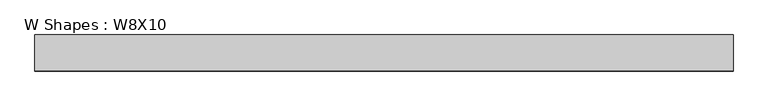
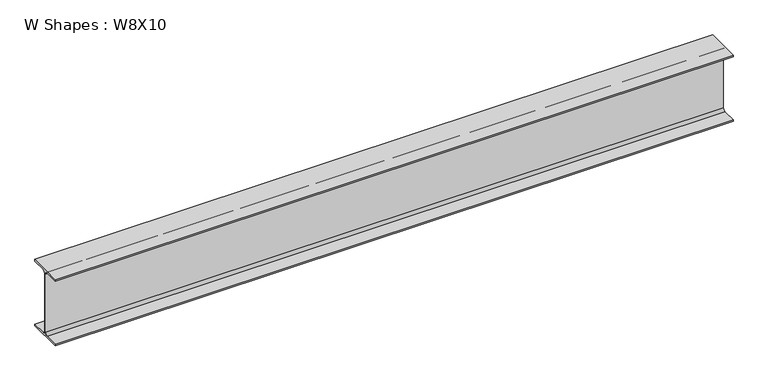
"""IFC4 building model written with IfcOpenShell, lengths in millimetres: beam geometry, W Shapes : W8X10."""

from ifc_helpers import new_model, si_unit, point, frame, frame_2d, origin, place, context, project, spatial, polyline, circle_curve, trimmed, segment, composite_curve, outline, extrude, source, transform, mapped, element, save


def w_shapes_w8x10_27fc2ad7(model_context):
    return source(origin(), model_context, "Body", "SweptSolid", [
        extrude(outline(composite_curve([segment(polyline([(50.038, -94.996), (50.038, -100.203), (-50.038, -100.203), (-50.038, -94.996), (-9.779, -94.996)]), True, "CONTINUOUS"), segment(trimmed(circle_curve(frame_2d((-9.779, -87.376)), 7.62), [point((-9.779, -94.996))], [point((-2.159, -87.376))], True, "CARTESIAN"), True, "CONTINUOUS"), segment(polyline([(-2.159, -87.376), (-2.159, 87.376)]), True, "CONTINUOUS"), segment(trimmed(circle_curve(frame_2d((-9.779, 87.376)), 7.62), [point((-2.159, 87.376))], [point((-9.779, 94.996))], True, "CARTESIAN"), True, "CONTINUOUS"), segment(polyline([(-9.779, 94.996), (-50.038, 94.996), (-50.038, 100.203), (50.038, 100.203), (50.038, 94.996), (9.779, 94.996)]), True, "CONTINUOUS"), segment(trimmed(circle_curve(frame_2d((9.779, 87.376)), 7.62), [point((9.779, 94.996))], [point((2.159, 87.376))], True, "CARTESIAN"), True, "CONTINUOUS"), segment(polyline([(2.159, 87.376), (2.159, -87.376)]), True, "CONTINUOUS"), segment(trimmed(circle_curve(frame_2d((9.779, -87.376)), 7.62), [point((2.159, -87.376))], [point((9.779, -94.996))], True, "CARTESIAN"), True, "CONTINUOUS"), segment(polyline([(9.779, -94.996), (50.038, -94.996)]), True, "CONTINUOUS")], self_intersect=False)), frame((-967.994, 0.0, 0.0), z_axis=(1.0, 0.0, 0.0), x_axis=(0.0, 1.0, 0.0)), (0.0, 0.0, 1.0), 1935.988),
    ])


if __name__ == "__main__":
    model = new_model("IFC4")
    model_context = context("Model", 3, world=origin())
    ifc_project = project(units=[si_unit("LENGTHUNIT", "METRE", prefix="MILLI")], contexts=[model_context])
    site = spatial("IfcSite", under=ifc_project)
    building = spatial("IfcBuilding", under=site)
    placement = place(None, origin())
    w_shapes_w8x10_shape = w_shapes_w8x10_27fc2ad7(model_context)
    element("IfcBeam", 1, ObjectType="W Shapes : W8X10", at=placement, inside=building, context=model_context, shape_type="MappedRepresentation", body=[
        mapped(w_shapes_w8x10_shape, transform((0.0, 0.0, 0.0), x_axis=(1.0, 0.0, 0.0), y_axis=(0.0, 1.0, 0.0), z_axis=(0.0, 0.0, 1.0))),
    ])
    save(model, "model.ifc")

# Revit data of these elements
# Type "W Shapes : W8X10"
#   Section Name Key = "W8x10"
#   Assembly Code = "B10"
#   Width = 3.940"
#   Web Thickness = 0.170"
#   Web Fillet = 0.300"
#   Warping Constant = 30.90 in⁶
#   Torsional Moment of Inertia = 0.0426 in⁴
#   Section Area = 2.96 in²
#   Plastic Modulus weak axis = 1.66 in³
#   Plastic Modulus strong axis = 8.87 in³
#   Perimeter = 30.70 ft²/ft
#   Nominal Weight = 10.00 lbf/ft
#   Moment of Inertia weak axis = 2.09 in⁴
#   Moment of Inertia strong axis = 30.80 in⁴
#   Height = 7.890"
#   Flange Thickness = 0.205"
#   Elastic Modulus weak axis = 1.06 in³
#   Elastic Modulus strong axis = 7.81 in³
#   Centroid Vertical = 3.945"
#   Centroid Horizontal = 1.970"
#   Bolt Spacing = 0' - 2 1/4"
#   Length [instance default] = 5' - 0"
#   Structural Material [instance default] = Steel ASTM A992
#   Principal Axes Angle = 0
# Element 1 (IfcBeam, "W Shapes : W8X10")
#   Materials on its faces: "Steel ASTM A992"
# Materials
#   "Steel ASTM A992": class "Metal", colour RGB 199 199 199, transparency 0, Description = "Structural steel 50ksi", Cost = 0
